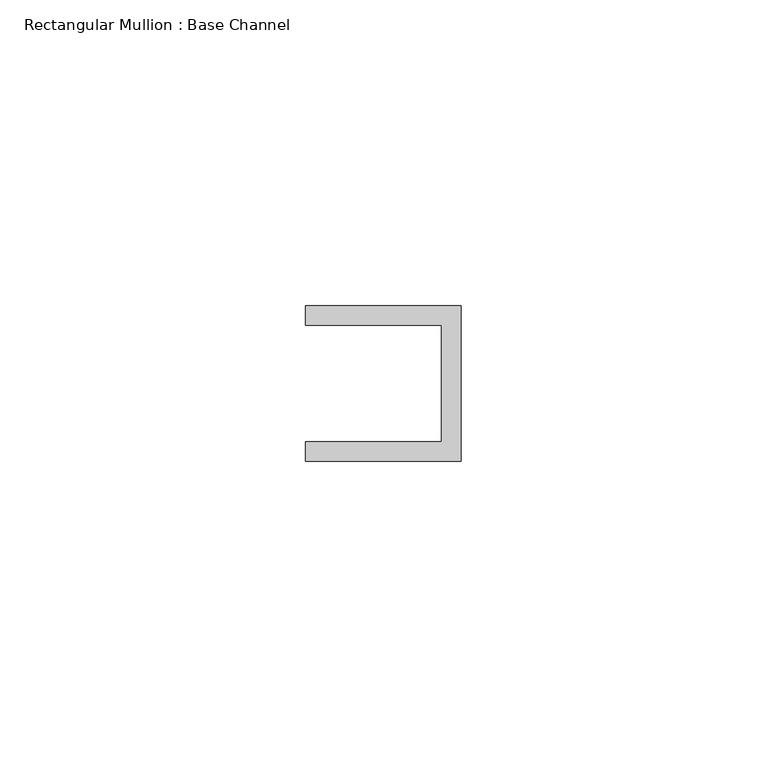
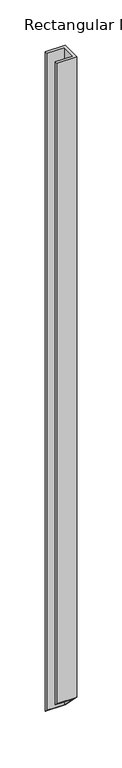
"""IFC4 building model written with IfcOpenShell, lengths in millimetres: member geometry, Rectangular Mullion : Base Channel."""

import ifcopenshell
import ifcopenshell.guid

model = None  # the IFC model being written
_history = None  # IfcOwnerHistory: only IFC2X3 demands one
_inside = {}  # id of a spatial element -> (the spatial element, [elements in it])
_under = {}  # id of a project, library or spatial element -> (it, [spatial elements below it])
_declared = {}  # id of a project -> (the project, [libraries it declares])
_typed = {}  # id of a type object -> (the type object, [elements of that type])
_made_of = {}  # id of a material, layer set ... -> (it, [elements and type objects made of it])


def new_model(schema):
    """Start an empty IFC model of exactly this schema.

    Asked for "IFC4X3", IfcOpenShell would pick the latest addendum, in which some entities
    have other attributes; the version numbers below select the first issue.
    IFC2X3 requires an IfcOwnerHistory on every rooted entity: one is made here for all.
    """
    global model, _history
    if schema == "IFC4X3":
        model = ifcopenshell.file(schema_version=(4, 3, 0, 0))
    else:
        model = ifcopenshell.file(schema=schema)
    _inside.clear()
    _under.clear()
    _declared.clear()
    _typed.clear()
    _made_of.clear()
    _history = None
    if model.schema == "IFC2X3":
        org = make("IfcOrganization", Name="unknown")
        user = make(
            "IfcPersonAndOrganization",
            ThePerson=make("IfcPerson", FamilyName="unknown"),
            TheOrganization=org,
        )
        app = make(
            "IfcApplication",
            ApplicationDeveloper=org,
            Version="unknown",
            ApplicationFullName="unknown",
            ApplicationIdentifier="unknown",
        )
        _history = make(
            "IfcOwnerHistory",
            OwningUser=user,
            OwningApplication=app,
            ChangeAction="ADDED",
            CreationDate=0,
        )
    return model


def make(cls, **values):
    """One entity of the class cls with the attributes given. An attribute that is None is left unset."""
    return model.create_entity(
        cls, **{name: value for name, value in values.items() if value is not None}
    )


def rooted(cls, **values):
    """An entity with a GlobalId (a new one), such as an element, a storey or a relation."""
    return make(cls, GlobalId=ifcopenshell.guid.new(), OwnerHistory=_history, **values)


def si_unit(unit_type, name, prefix=None):
    """IfcSIUnit, for example si_unit("LENGTHUNIT", "METRE", prefix="MILLI")."""
    return make("IfcSIUnit", UnitType=unit_type, Prefix=prefix, Name=name)


def assignment(units):
    """IfcUnitAssignment: the units of a project."""
    return None if units is None else make("IfcUnitAssignment", Units=units)


def point(xyz):
    """IfcCartesianPoint."""
    return None if xyz is None else make("IfcCartesianPoint", Coordinates=xyz)


def direction(xyz):
    """IfcDirection."""
    return None if xyz is None else make("IfcDirection", DirectionRatios=xyz)


def frame(location, z_axis=None, x_axis=None):
    """IfcAxis2Placement3D, a coordinate frame: its origin and axes. An axis left out is left unset."""
    return make(
        "IfcAxis2Placement3D",
        Location=point(location),
        Axis=direction(z_axis),
        RefDirection=direction(x_axis),
    )


def origin():
    """The frame at (0, 0, 0) with its axes left unset."""
    return frame((0.0, 0.0, 0.0))


def place(relative_to, where):
    """IfcLocalPlacement: puts the frame where relative to a parent placement (None: the world)."""
    return make(
        "IfcLocalPlacement", PlacementRelTo=relative_to, RelativePlacement=where
    )


def context(
    kind, dimensions, precision=None, world=None, true_north=None, identifier=None
):
    """IfcGeometricRepresentationContext, for example the 3D "Model" context."""
    return make(
        "IfcGeometricRepresentationContext",
        ContextIdentifier=identifier,
        ContextType=kind,
        CoordinateSpaceDimension=dimensions,
        Precision=precision,
        WorldCoordinateSystem=world,
        TrueNorth=true_north,
    )


def project(units=None, contexts=None):
    """IfcProject with its units and contexts."""
    return rooted(
        "IfcProject",
        Name="project",
        RepresentationContexts=contexts,
        UnitsInContext=assignment(units),
    )


def spatial(cls, under=None, at=None, **own):
    """A site, building, storey or space (cls), placed at a placement, below another one or the project."""
    s = rooted(cls, ObjectPlacement=at, **own)
    if under is not None:
        _under.setdefault(under.id(), (under, []))[1].append(s)
    return s


def faces_of(points, faces, orient=None, outer=None):
    """IfcFace entities. A face is a list of loops; a loop is a list of indices into points, from 0.

    orient and outer hold one flag for each loop. By default every Orientation is true, the
    first loop of a face is its IfcFaceOuterBound and the others are IfcFaceBound.
    """
    made = []
    for i, loops in enumerate(faces):
        bounds = []
        for j, loop in enumerate(loops):
            is_outer = j == 0 if outer is None else outer[i][j]
            bounds.append(
                make(
                    "IfcFaceOuterBound" if is_outer else "IfcFaceBound",
                    Bound=make("IfcPolyLoop", Polygon=[points[k] for k in loop]),
                    Orientation=True if orient is None else orient[i][j],
                )
            )
        made.append(make("IfcFace", Bounds=bounds))
    return made


def faceted_brep(points, faces, orient=None, outer=None, voids=None):
    """IfcFacetedBrep: a solid bounded by flat faces; with voids (closed shells), ...WithVoids."""
    shared = [point(p) for p in points]
    hull = make("IfcClosedShell", CfsFaces=faces_of(shared, faces, orient, outer))
    if voids is None:
        return make("IfcFacetedBrep", Outer=hull)
    return make(
        "IfcFacetedBrepWithVoids",
        Outer=hull,
        Voids=[
            make(cls, CfsFaces=faces_of(shared, fs, o, b)) for cls, fs, o, b in voids
        ],
    )


def shape(context_of_items, identifier, shape_type, items):
    """IfcShapeRepresentation: the items that make up one representation, for example the "Body"."""
    return make(
        "IfcShapeRepresentation",
        ContextOfItems=context_of_items,
        RepresentationIdentifier=identifier,
        RepresentationType=shape_type,
        Items=items,
    )


def source(mapping_origin, context_of_items, identifier, shape_type, items):
    """IfcRepresentationMap: a shape defined once, which mapped items show again and again."""
    return make(
        "IfcRepresentationMap",
        MappingOrigin=mapping_origin,
        MappedRepresentation=shape(context_of_items, identifier, shape_type, items),
    )


def transform(
    local_origin,
    x_axis=None,
    y_axis=None,
    z_axis=None,
    scale=None,
    scale2=None,
    scale3=None,
    uniform=True,
):
    """IfcCartesianTransformationOperator3D, or its non-uniform kind. x_axis, y_axis, z_axis: its Axis1, 2, 3."""
    if uniform:
        return make(
            "IfcCartesianTransformationOperator3D",
            Axis1=direction(x_axis),
            Axis2=direction(y_axis),
            LocalOrigin=point(local_origin),
            Scale=scale,
            Axis3=direction(z_axis),
        )
    return make(
        "IfcCartesianTransformationOperator3DnonUniform",
        Axis1=direction(x_axis),
        Axis2=direction(y_axis),
        LocalOrigin=point(local_origin),
        Scale=scale,
        Axis3=direction(z_axis),
        Scale2=scale2,
        Scale3=scale3,
    )


def mapped(mapping_source, mapping_target):
    """IfcMappedItem: shows the shape of a source again, moved by a transform."""
    return make(
        "IfcMappedItem", MappingSource=mapping_source, MappingTarget=mapping_target
    )


def made_of(thing, what):
    """Note that an element or type object is made of a material, layer set ...; save() writes the relation."""
    if what is not None:
        _made_of.setdefault(what.id(), (what, []))[1].append(thing)
    return thing


def element(
    cls,
    number,
    at=None,
    inside=None,
    cuts=None,
    type_object=None,
    material=None,
    context=None,
    identifier="Body",
    shape_type=None,
    held_by="IfcProductDefinitionShape",
    body=None,
    shapes=None,
    **own,
):
    """One element of the class cls, such as IfcWall. Its Tag is "e" and its number.

    at: its placement. inside: the storey or other place that contains it. cuts: it is an
    opening in that element (IfcRelVoidsElement). A single representation is given by context,
    identifier, shape_type and body (its items); several are given by shapes. held_by: the class
    of the entity that holds the representations. save() writes the other relations.
    """
    e = rooted(cls, Tag="e%d" % number, ObjectPlacement=at, **own)
    if body is not None:
        shapes = [shape(context, identifier, shape_type, body)]
    if shapes is not None:
        e.Representation = make(held_by, Representations=shapes)
    if inside is not None:
        _inside.setdefault(inside.id(), (inside, []))[1].append(e)
    if cuts is not None:
        rooted(
            "IfcRelVoidsElement", RelatingBuildingElement=cuts, RelatedOpeningElement=e
        )
    if type_object is not None:
        _typed.setdefault(type_object.id(), (type_object, []))[1].append(e)
    return made_of(e, material)


def aggregate(whole, parts):
    """IfcRelAggregates: a whole, such as a stair, and the parts it consists of."""
    return rooted("IfcRelAggregates", RelatingObject=whole, RelatedObjects=parts)


def save(model, path):
    """Write the relations noted so far, then the file.

    IfcRelAggregates (storeys below a building ...), IfcRelContainedInSpatialStructure (elements
    in a storey), IfcRelDefinesByType, IfcRelAssociatesMaterial and IfcRelDeclares: one each for
    every whole, place, type object, material and project.
    """
    for whole, parts in _under.values():
        aggregate(whole, parts)
    for where, things in _inside.values():
        rooted(
            "IfcRelContainedInSpatialStructure",
            RelatedElements=things,
            RelatingStructure=where,
        )
    for kind, things in _typed.values():
        rooted("IfcRelDefinesByType", RelatedObjects=things, RelatingType=kind)
    for what, things in _made_of.values():
        rooted("IfcRelAssociatesMaterial", RelatedObjects=things, RelatingMaterial=what)
    for by, libraries in _declared.values():
        rooted("IfcRelDeclares", RelatingContext=by, RelatedDefinitions=libraries)
    model.write(path)


def rectangular_mullion_base_channel_91f86e7e(model_context):
    return source(origin(), model_context, "Body", "Brep", [
        faceted_brep([(0.0, 12.7, 0.0), (-25.4, 12.7, 0.0), (-25.4, 9.525, 0.0), (-3.175, 9.525, 0.0), (-3.175, -9.525, 0.0), (-25.4, -9.525, 0.0), (-25.4, -12.7, 0.0), (0.0, -12.7, 0.0), (0.0, 12.7, -889.3175002), (-25.4, 12.7, -889.3175002), (-25.4, 9.525, -886.1425002), (-3.175, 9.525, -886.1425002), (-3.175, -9.525, -867.0925002), (-25.4, -9.525, -867.0925002), (-25.4, -12.7, -863.9175002), (0.0, -12.7, -863.9175002)], [[[0, 1, 2, 3, 4, 5, 6, 7]], [[1, 0, 8, 9]], [[2, 1, 9, 10]], [[3, 2, 10, 11]], [[4, 3, 11, 12]], [[5, 4, 12, 13]], [[6, 5, 13, 14]], [[7, 6, 14, 15]], [[0, 7, 15, 8]], [[8, 15, 14, 13, 12, 11, 10, 9]]]),
    ])


if __name__ == "__main__":
    model = new_model("IFC4")
    model_context = context("Model", 3, world=origin())
    ifc_project = project(units=[si_unit("LENGTHUNIT", "METRE", prefix="MILLI")], contexts=[model_context])
    site = spatial("IfcSite", under=ifc_project)
    building = spatial("IfcBuilding", under=site)
    placement = place(None, origin())
    rectangular_mullion_base_channel_shape = rectangular_mullion_base_channel_91f86e7e(model_context)
    element("IfcMember", 1, ObjectType="Rectangular Mullion : Base Channel", at=placement, inside=building, context=model_context, shape_type="MappedRepresentation", body=[
        mapped(rectangular_mullion_base_channel_shape, transform((0.0, 0.0, 0.0), x_axis=(1.0, 0.0, 0.0), y_axis=(0.0, 1.0, 0.0), z_axis=(0.0, 0.0, 1.0))),
    ])
    save(model, "model.ifc")

# Revit data of these elements
# Type "Rectangular Mullion : Base Channel"
#   built-in parameter 1007322 = 0.0833333 (stored number, unit not read)
#   built-in parameter 1007321 = 0.0416667 (stored number, unit not read)
#   built-in parameter 1007320 = -0.03125 (stored number, unit not read)
# Element 1 (IfcMember, "Rectangular Mullion : Base Channel")
#   Materials on its faces: "ALUM"
# Materials
#   "ALUM": class "Generic", colour RGB 157 157 157, transparency 0, Cost = 0
